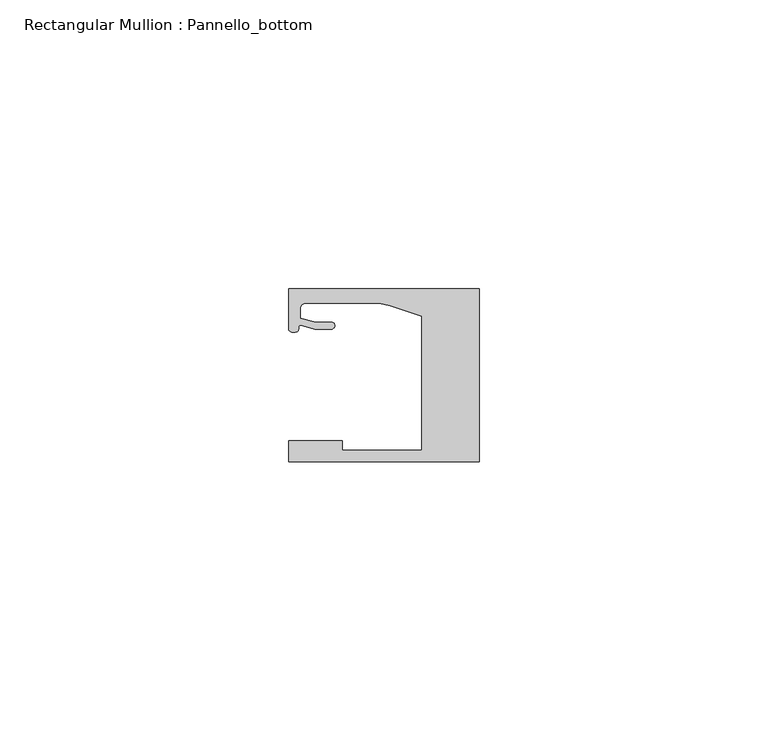
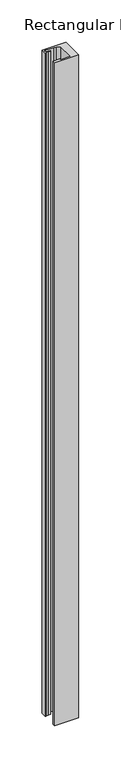
"""IFC4 building model written with IfcOpenShell, lengths in millimetres: member geometry, Rectangular Mullion : Pannello_bottom."""

from ifc_helpers import new_model, si_unit, frame, origin, place, context, project, spatial, polyline, circle_curve, source, transform, mapped, element, save
from ifc_brep_helpers import plane_surface, cylinder_surface, revolved_surface, extruded_surface, spline_curve, advanced_brep


def rectangular_mullion_pannello_bottom_56fb9db7(model_context):
    return source(origin(), model_context, "Body", "AdvancedBrep", [
        advanced_brep(
        [(-33.0, -15.0, 0.0), (0.0, -15.0, 0.0), (0.0, 15.0, 0.0), (-33.0000135, 15.0, 0.0), (-33.0000135, 8.0000472, 0.0), (-30.9223017, 8.6490241, 0.0), (-28.4999305, 7.9999523, 0.0), (-25.59998, 7.9999523, 0.0), (-25.59998, 9.1999523, 0.0), (-28.3419477, 9.1999523, 0.0), (-31.0, 9.9121746, 0.0), (-31.0, 11.4999419, 0.0), (-30.0000002, 12.4999419, 0.0), (-18.5493024, 12.4999438, 0.0), (-15.4591336, 12.0105099, 0.0), (-9.9999723, 10.2367227, 0.0), (-9.9999723, -13.0000004, 0.0), (-23.700041, -13.0000004, 0.0), (-23.700041, -11.3000004, 0.0), (-33.0, -11.3000004, 0.0), (-33.0, -15.0, -960.0), (-33.0, -11.3000004, -960.0), (-23.700041, -11.3000004, -960.0), (-23.700041, -13.0000004, -960.0), (-9.9999723, -13.0000004, -960.0), (-9.9999723, 10.2367227, -960.0), (-15.4591336, 12.0105099, -960.0), (-18.5493024, 12.4999438, -960.0), (-30.0000002, 12.4999419, -960.0), (-31.0, 11.4999419, -960.0), (-31.0, 9.9121746, -960.0), (-28.3419477, 9.1999523, -960.0), (-25.59998, 9.1999523, -960.0), (-25.59998, 7.9999523, -960.0), (-28.4999305, 7.9999523, -960.0), (-30.9223017, 8.6490241, -960.0), (-33.0000135, 8.0000472, -960.0), (-33.0000135, 15.0, -960.0), (0.0, 15.0, -960.0), (0.0, -15.0, -960.0)],
        [
            (0, 1),
            (1, 2),
            (2, 3),
            (3, 4),
            (4, 5, spline_curve(3, [(-33.0000135, 8.0000472, 0.0), (-33.0000135, 7.457047519, 0.0), (-32.262327879, 7.456527435, 0.0), (-31.357433266, 7.563996614, 0.0), (-31.305645054, 7.690065204, 0.0), (-31.298563602, 8.366228555, 0.0), (-31.312054066, 8.717747958, 0.0), (-30.9223017, 8.6490241, 0.0)], [4, 2, 2, 4], [0.0, 0.0027053965905959043, 0.0058611956533709, 0.007702013405570312])),
            (5, 6),
            (6, 7),
            (7, 8, circle_curve(frame((-25.59998, 8.5999523, 0.0), z_axis=(0.0, 0.0, 1.0), x_axis=(0.0, 1.0, 0.0)), 0.6)),
            (8, 9),
            (9, 10),
            (10, 11),
            (11, 12, circle_curve(frame((-30.0, 11.4999419, 0.0), z_axis=(0.0, 0.0, -1.0), x_axis=(0.0, 1.0, 0.0)), 1.0)),
            (12, 13),
            (13, 14, circle_curve(frame((-18.5493007, 2.4999438, 0.0), z_axis=(0.0, 0.0, -1.0), x_axis=(0.0, 1.0, 0.0)), 10.0)),
            (14, 15),
            (15, 16),
            (16, 17),
            (17, 18),
            (18, 19),
            (19, 0),
            (20, 21),
            (21, 22),
            (22, 23),
            (23, 24),
            (24, 25),
            (25, 26),
            (26, 27, circle_curve(frame((-18.5493007, 2.4999438, -960.0), z_axis=(0.0, 0.0, 1.0), x_axis=(0.0, 1.0, 0.0)), 10.0)),
            (27, 28),
            (28, 29, circle_curve(frame((-30.0, 11.4999419, -960.0), z_axis=(0.0, 0.0, 1.0), x_axis=(0.0, 1.0, 0.0)), 1.0)),
            (29, 30),
            (30, 31),
            (31, 32),
            (32, 33, circle_curve(frame((-25.59998, 8.5999523, -960.0), z_axis=(0.0, 0.0, -1.0), x_axis=(0.0, 1.0, 0.0)), 0.6)),
            (33, 34),
            (34, 35),
            (35, 36, spline_curve(3, [(-30.9223017, 8.6490241, -960.0), (-31.312054066, 8.717747958, -960.0), (-31.298563602, 8.366228555, -960.0), (-31.305645054, 7.690065204, -960.0), (-31.357433266, 7.563996614, -960.0), (-32.262327879, 7.456527435, -960.0), (-33.0000135, 7.457047519, -960.0), (-33.0000135, 8.0000472, -960.0)], [4, 2, 2, 4], [0.0, 0.001840817752199412, 0.004996616814974408, 0.007702013405570312])),
            (36, 37),
            (37, 38),
            (38, 39),
            (39, 20),
            (0, 20),
            (39, 1),
            (38, 2),
            (37, 3),
            (36, 4),
            (35, 5),
            (34, 6),
            (33, 7),
            (32, 8),
            (31, 9),
            (30, 10),
            (29, 11),
            (28, 12),
            (27, 13),
            (26, 14),
            (25, 15),
            (24, 16),
            (23, 17),
            (22, 18),
            (21, 19),
        ],
        [
            plane_surface(frame((0.0, -36.2491502, 0.0), z_axis=(0.0, 0.0, 1.0), x_axis=(-1.0, 0.0, 0.0))),
            plane_surface(frame((0.0, -36.2491502, -960.0), z_axis=(0.0, 0.0, -1.0), x_axis=(-1.0, 0.0, 0.0))),
            plane_surface(frame((-33.0, -15.0, 0.0), z_axis=(0.0, -1.0, 0.0), x_axis=(0.0, 0.0, -1.0))),
            plane_surface(frame((0.0, -15.0, 0.0), z_axis=(1.0, 0.0, 0.0), x_axis=(0.0, 0.0, -1.0))),
            plane_surface(frame((0.0, 15.0, 0.0), z_axis=(0.0, 1.0, 0.0), x_axis=(0.0, 0.0, -1.0))),
            plane_surface(frame((-33.0000135, 15.0, 0.0), z_axis=(-1.0, 0.0, 0.0), x_axis=(0.0, 0.0, -1.0))),
            extruded_surface(spline_curve(3, [(-33.0000135, 8.0000472, -960.0), (-33.0000135, 7.457047519, -960.0), (-32.262327879, 7.456527435, -960.0), (-31.357433266, 7.563996614, -960.0), (-31.305645054, 7.690065204, -960.0), (-31.298563602, 8.366228555, -960.0), (-31.312054066, 8.717747958, -960.0), (-30.9223017, 8.6490241, -960.0)], [4, 2, 2, 4], [0.0, 0.0027053965905959043, 0.0058611956533709, 0.007702013405570312]), (0.0, 0.0, 960.0), 960.0),
            plane_surface(frame((-30.9223017, 8.6490241, 0.0), z_axis=(-0.25881883200192934, -0.9659258833891746, 0.0), x_axis=(0.0, 0.0, -1.0))),
            plane_surface(frame((-28.4999305, 7.9999523, 0.0), z_axis=(0.0, -1.0, 0.0), x_axis=(0.0, 0.0, -1.0))),
            cylinder_surface(frame((-25.59998, 8.5999523, 0.0), z_axis=(0.0, 0.0, 1.0), x_axis=(0.0, 1.0, 0.0)), 0.6),
            plane_surface(frame((-25.59998, 9.1999523, 0.0), z_axis=(0.0, 1.0, 0.0), x_axis=(0.0, 0.0, -1.0))),
            plane_surface(frame((-28.3419477, 9.1999523, 0.0), z_axis=(0.25881883204288636, 0.9659258833782002, 0.0), x_axis=(0.0, 0.0, -1.0))),
            plane_surface(frame((-31.0, 9.9121746, 0.0), z_axis=(1.0, 0.0, 0.0), x_axis=(0.0, 0.0, -1.0))),
            revolved_surface(polyline([(-30.0, 12.4999419, -960.0), (-30.0, 12.4999419, 0.0)]), (-30.0, 11.4999419, 0.0), (0.0, 0.0, -1.0)),
            plane_surface(frame((-30.0000002, 12.4999419, 0.0), z_axis=(1.6923026533778639e-07, -0.9999999999999858, 0.0), x_axis=(0.0, 0.0, -1.0))),
            revolved_surface(polyline([(-18.5493007, 12.4999438, -960.0), (-18.5493007, 12.4999438, 0.0)]), (-18.5493007, 2.4999438, 0.0), (0.0, 0.0, -1.0)),
            plane_surface(frame((-15.4591336, 12.0105099, 0.0), z_axis=(-0.30901670911956314, -0.9510566089801992, 0.0), x_axis=(0.0, 0.0, -1.0))),
            plane_surface(frame((-9.9999723, 10.2367227, 0.0), z_axis=(-1.0, 0.0, 0.0), x_axis=(0.0, 0.0, -1.0))),
            plane_surface(frame((-9.9999723, -13.0000004, 0.0), z_axis=(0.0, 1.0, 0.0), x_axis=(0.0, 0.0, -1.0))),
            plane_surface(frame((-23.700041, -13.0000004, 0.0), z_axis=(1.0, 0.0, 0.0), x_axis=(0.0, 0.0, -1.0))),
            plane_surface(frame((-23.700041, -11.3000004, 0.0), z_axis=(0.0, 1.0, 0.0), x_axis=(0.0, 0.0, -1.0))),
            plane_surface(frame((-33.0, -11.3000004, 0.0), z_axis=(-1.0, 0.0, 0.0), x_axis=(0.0, 0.0, -1.0))),
        ],
        [
            (0, [[1, 2, 3, 4, 5, 6, 7, 8, 9, 10, 11, 12, 13, 14, 15, 16, 17, 18, 19, 20]]),
            (1, [[21, 22, 23, 24, 25, 26, 27, 28, 29, 30, 31, 32, 33, 34, 35, 36, 37, 38, 39, 40]]),
            (2, [[-1, 41, -40, 42]]),
            (3, [[-2, -42, -39, 43]]),
            (4, [[-3, -43, -38, 44]]),
            (5, [[-4, -44, -37, 45]]),
            (6, [[-5, -45, -36, 46]]),
            (7, [[-6, -46, -35, 47]]),
            (8, [[-7, -47, -34, 48]]),
            (9, [[-8, -48, -33, 49]]),
            (10, [[-9, -49, -32, 50]]),
            (11, [[-10, -50, -31, 51]]),
            (12, [[-11, -51, -30, 52]]),
            (13, [[-12, -52, -29, 53]]),
            (14, [[-13, -53, -28, 54]]),
            (15, [[-14, -54, -27, 55]]),
            (16, [[-15, -55, -26, 56]]),
            (17, [[-16, -56, -25, 57]]),
            (18, [[-17, -57, -24, 58]]),
            (19, [[-18, -58, -23, 59]]),
            (20, [[-19, -59, -22, 60]]),
            (21, [[-20, -60, -21, -41]]),
        ],
    ),
    ])


if __name__ == "__main__":
    model = new_model("IFC4")
    model_context = context("Model", 3, world=origin())
    ifc_project = project(units=[si_unit("LENGTHUNIT", "METRE", prefix="MILLI")], contexts=[model_context])
    site = spatial("IfcSite", under=ifc_project)
    building = spatial("IfcBuilding", under=site)
    placement = place(None, origin())
    rectangular_mullion_pannello_bottom_shape = rectangular_mullion_pannello_bottom_56fb9db7(model_context)
    element("IfcMember", 1, ObjectType="Rectangular Mullion : Pannello_bottom", at=placement, inside=building, context=model_context, shape_type="MappedRepresentation", body=[
        mapped(rectangular_mullion_pannello_bottom_shape, transform((0.0, 0.0, 0.0), x_axis=(1.0, 0.0, 0.0), y_axis=(0.0, 1.0, 0.0), z_axis=(0.0, 0.0, 1.0))),
    ])
    save(model, "model.ifc")

# Revit data of these elements
# Type "Rectangular Mullion : Pannello_bottom"
#   built-in parameter 1007322 = 0.0984252 (stored number, unit not read)
#   built-in parameter 1007321 = 0.0328083 (stored number, unit not read)
#   built-in parameter 1007320 = 0 (stored number, unit not read)
